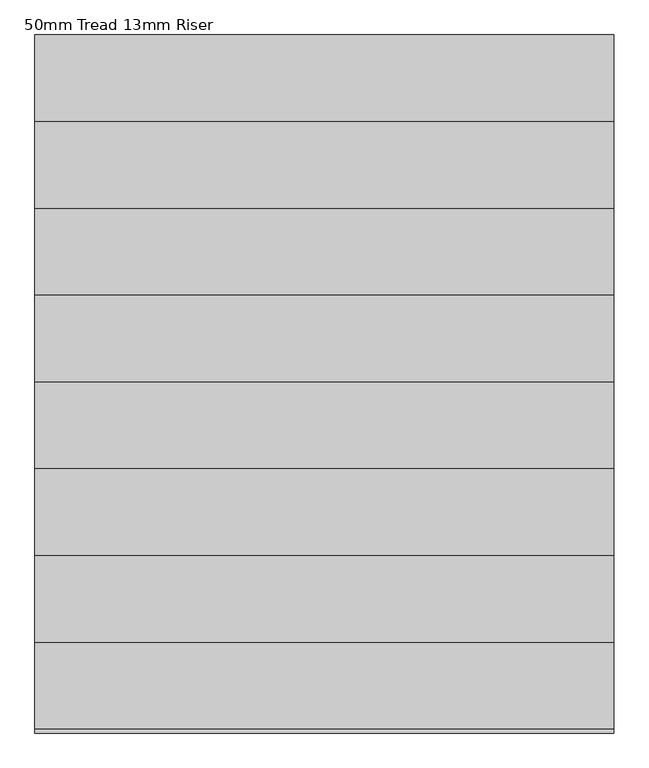
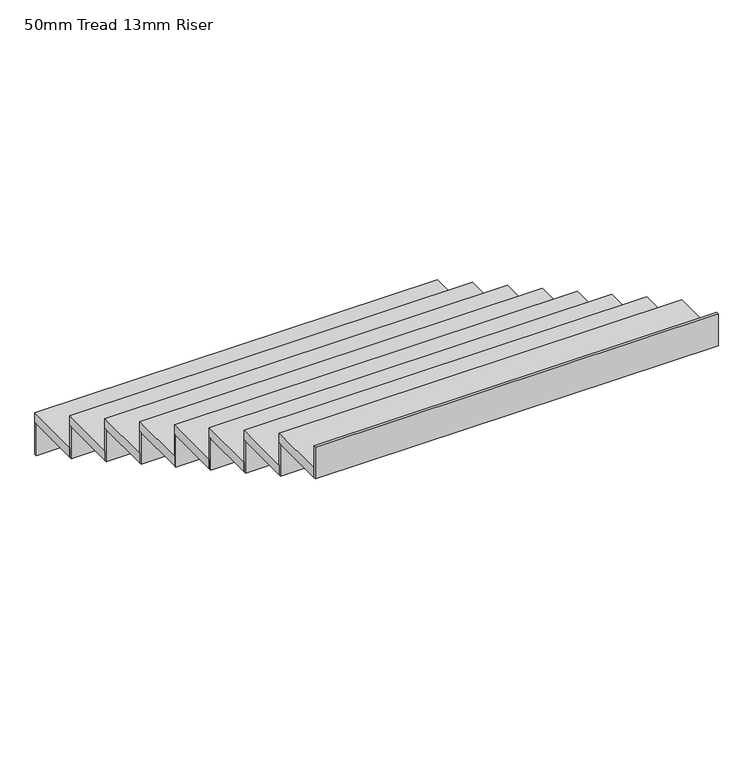
"""IFC4 building model written with IfcOpenShell, lengths in millimetres: stair flight geometry, 50mm Tread 13mm Riser."""

from ifc_helpers import new_model, si_unit, frame, origin, place, context, project, spatial, polyline, outline, extrude, source, transform, mapped, element, save


def stair_flight_50mm_tread_13mm_riser_7dc9fb9b(model_context):
    return source(origin(), model_context, "Body", "SweptSolid", [
        extrude(outline(polyline([(15000.0002442, 23517.4999999), (15000.0002442, 23529.9999999), (17000.0002442, 23529.9999999), (17000.0002442, 23517.4999999), (15000.0002442, 23517.4999999)])), frame((0.0, 0.0, 30450.0), z_axis=(0.0, 0.0, 1.0), x_axis=(1.0, 0.0, 0.0)), (0.0, 0.0, 1.0), 166.6666667),
        extrude(outline(polyline([(17000.0002442, 23229.9999999), (15000.0002442, 23229.9999999), (15000.0002442, 23529.9999999), (17000.0002442, 23529.9999999), (17000.0002442, 23229.9999999)])), frame((0.0, 0.0, 30616.6666667), z_axis=(0.0, 0.0, 1.0), x_axis=(1.0, 0.0, 0.0)), (0.0, 0.0, 1.0), 50.0),
        extrude(outline(polyline([(15000.0002442, 23217.4999999), (15000.0002442, 23229.9999999), (17000.0002442, 23229.9999999), (17000.0002442, 23217.4999999), (15000.0002442, 23217.4999999)])), frame((0.0, 0.0, 30616.6666667), z_axis=(0.0, 0.0, 1.0), x_axis=(1.0, 0.0, 0.0)), (0.0, 0.0, 1.0), 166.6666667),
        extrude(outline(polyline([(17000.0002442, 22929.9999999), (15000.0002442, 22929.9999999), (15000.0002442, 23229.9999999), (17000.0002442, 23229.9999999), (17000.0002442, 22929.9999999)])), frame((0.0, 0.0, 30783.3333333), z_axis=(0.0, 0.0, 1.0), x_axis=(1.0, 0.0, 0.0)), (0.0, 0.0, 1.0), 50.0),
        extrude(outline(polyline([(15000.0002442, 22917.4999999), (15000.0002442, 22929.9999999), (17000.0002442, 22929.9999999), (17000.0002442, 22917.4999999), (15000.0002442, 22917.4999999)])), frame((0.0, 0.0, 30783.3333333), z_axis=(0.0, 0.0, 1.0), x_axis=(1.0, 0.0, 0.0)), (0.0, 0.0, 1.0), 166.6666667),
        extrude(outline(polyline([(17000.0002442, 22629.9999999), (15000.0002442, 22629.9999999), (15000.0002442, 22929.9999999), (17000.0002442, 22929.9999999), (17000.0002442, 22629.9999999)])), frame((0.0, 0.0, 30950.0), z_axis=(0.0, 0.0, 1.0), x_axis=(1.0, 0.0, 0.0)), (0.0, 0.0, 1.0), 50.0),
        extrude(outline(polyline([(15000.0002442, 22617.4999999), (15000.0002442, 22629.9999999), (17000.0002442, 22629.9999999), (17000.0002442, 22617.4999999), (15000.0002442, 22617.4999999)])), frame((0.0, 0.0, 30950.0), z_axis=(0.0, 0.0, 1.0), x_axis=(1.0, 0.0, 0.0)), (0.0, 0.0, 1.0), 166.6666667),
        extrude(outline(polyline([(17000.0002442, 22329.9999999), (15000.0002442, 22329.9999999), (15000.0002442, 22629.9999999), (17000.0002442, 22629.9999999), (17000.0002442, 22329.9999999)])), frame((0.0, 0.0, 31116.6666667), z_axis=(0.0, 0.0, 1.0), x_axis=(1.0, 0.0, 0.0)), (0.0, 0.0, 1.0), 50.0),
        extrude(outline(polyline([(15000.0002442, 22317.4999999), (15000.0002442, 22329.9999999), (17000.0002442, 22329.9999999), (17000.0002442, 22317.4999999), (15000.0002442, 22317.4999999)])), frame((0.0, 0.0, 31116.6666667), z_axis=(0.0, 0.0, 1.0), x_axis=(1.0, 0.0, 0.0)), (0.0, 0.0, 1.0), 166.6666667),
        extrude(outline(polyline([(17000.0002442, 22029.9999999), (15000.0002442, 22029.9999999), (15000.0002442, 22329.9999999), (17000.0002442, 22329.9999999), (17000.0002442, 22029.9999999)])), frame((0.0, 0.0, 31283.3333333), z_axis=(0.0, 0.0, 1.0), x_axis=(1.0, 0.0, 0.0)), (0.0, 0.0, 1.0), 50.0),
        extrude(outline(polyline([(15000.0002442, 22017.4999999), (15000.0002442, 22029.9999999), (17000.0002442, 22029.9999999), (17000.0002442, 22017.4999999), (15000.0002442, 22017.4999999)])), frame((0.0, 0.0, 31283.3333333), z_axis=(0.0, 0.0, 1.0), x_axis=(1.0, 0.0, 0.0)), (0.0, 0.0, 1.0), 166.6666667),
        extrude(outline(polyline([(17000.0002442, 21729.9999999), (15000.0002442, 21729.9999999), (15000.0002442, 22029.9999999), (17000.0002442, 22029.9999999), (17000.0002442, 21729.9999999)])), frame((0.0, 0.0, 31450.0), z_axis=(0.0, 0.0, 1.0), x_axis=(1.0, 0.0, 0.0)), (0.0, 0.0, 1.0), 50.0),
        extrude(outline(polyline([(15000.0002442, 21717.4999999), (15000.0002442, 21729.9999999), (17000.0002442, 21729.9999999), (17000.0002442, 21717.4999999), (15000.0002442, 21717.4999999)])), frame((0.0, 0.0, 31450.0), z_axis=(0.0, 0.0, 1.0), x_axis=(1.0, 0.0, 0.0)), (0.0, 0.0, 1.0), 166.6666667),
        extrude(outline(polyline([(17000.0002442, 21429.9999999), (15000.0002442, 21429.9999999), (15000.0002442, 21729.9999999), (17000.0002442, 21729.9999999), (17000.0002442, 21429.9999999)])), frame((0.0, 0.0, 31616.6666667), z_axis=(0.0, 0.0, 1.0), x_axis=(1.0, 0.0, 0.0)), (0.0, 0.0, 1.0), 50.0),
        extrude(outline(polyline([(15000.0002442, 21417.4999999), (15000.0002442, 21429.9999999), (17000.0002442, 21429.9999999), (17000.0002442, 21417.4999999), (15000.0002442, 21417.4999999)])), frame((0.0, 0.0, 31616.6666667), z_axis=(0.0, 0.0, 1.0), x_axis=(1.0, 0.0, 0.0)), (0.0, 0.0, 1.0), 166.6666667),
        extrude(outline(polyline([(15000.0002442, 21117.4999999), (15000.0002442, 21129.9999999), (17000.0002442, 21129.9999999), (17000.0002442, 21117.4999999), (15000.0002442, 21117.4999999)])), frame((0.0, 0.0, 31783.3333333), z_axis=(0.0, 0.0, 1.0), x_axis=(1.0, 0.0, 0.0)), (0.0, 0.0, 1.0), 166.6666667),
        extrude(outline(polyline([(17000.0002442, 21129.9999999), (15000.0002442, 21129.9999999), (15000.0002442, 21429.9999999), (17000.0002442, 21429.9999999), (17000.0002442, 21129.9999999)])), frame((0.0, 0.0, 31783.3333333), z_axis=(0.0, 0.0, 1.0), x_axis=(1.0, 0.0, 0.0)), (0.0, 0.0, 1.0), 50.0),
    ])


if __name__ == "__main__":
    model = new_model("IFC4")
    model_context = context("Model", 3, world=origin())
    ifc_project = project(units=[si_unit("LENGTHUNIT", "METRE", prefix="MILLI")], contexts=[model_context])
    site = spatial("IfcSite", under=ifc_project)
    building = spatial("IfcBuilding", under=site)
    placement = place(None, origin())
    stair_flight_50mm_tread_13mm_riser_shape = stair_flight_50mm_tread_13mm_riser_7dc9fb9b(model_context)
    element("IfcStairFlight", 1, ObjectType="50mm Tread 13mm Riser", at=placement, inside=building, context=model_context, shape_type="MappedRepresentation", body=[
        mapped(stair_flight_50mm_tread_13mm_riser_shape, transform((0.0, 0.0, 0.0), x_axis=(1.0, 0.0, 0.0), y_axis=(0.0, 1.0, 0.0), z_axis=(0.0, 0.0, 1.0))),
    ])
    save(model, "model.ifc")
